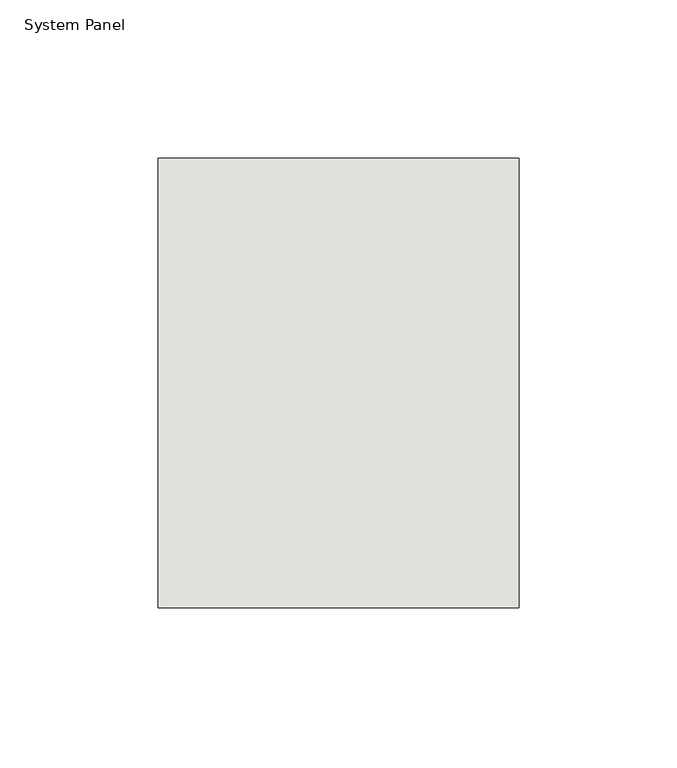
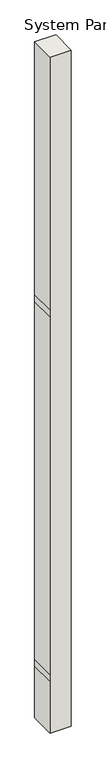
"""IFC4 building model written with IfcOpenShell, lengths in millimetres: wall geometry, System Panel : NLRS_21_CWP_hsb-vulling minerale wol 142 _gen_rsf."""

from ifc_helpers import new_model, si_unit, frame, origin, place, context, project, spatial, polyline, outline, extrude, source, transform, mapped, element, save


def system_panel_2185679e(model_context):
    return source(origin(), model_context, "Body", "SweptSolid", [
        extrude(outline(polyline([(0.0, -56.9999998), (0.0, 56.9999998), (295.0, 56.9999998), (333.0, 56.9999998), (2371.0, 56.9999998), (2409.0, 56.9999998), (3849.0, 56.9999998), (3849.0, -56.9999998), (2409.0, -56.9999998), (2371.0, -56.9999998), (333.0, -56.9999998), (295.0, -56.9999998), (0.0, -56.9999998)])), frame((0.0, -71.0, 0.0), z_axis=(0.0, 1.0, 0.0), x_axis=(0.0, 0.0, 1.0)), (0.0, 0.0, 1.0), 142.0),
    ])


if __name__ == "__main__":
    model = new_model("IFC4")
    model_context = context("Model", 3, world=origin())
    ifc_project = project(units=[si_unit("LENGTHUNIT", "METRE", prefix="MILLI")], contexts=[model_context])
    site = spatial("IfcSite", under=ifc_project)
    building = spatial("IfcBuilding", under=site)
    placement = place(None, origin())
    system_panel_shape = system_panel_2185679e(model_context)
    element("IfcWall", 1, ObjectType="System Panel : NLRS_21_CWP_hsb-vulling minerale wol 142 _gen_rsf", at=placement, inside=building, context=model_context, shape_type="MappedRepresentation", body=[
        mapped(system_panel_shape, transform((0.0, 0.0, 0.0), x_axis=(1.0, 0.0, 0.0), y_axis=(0.0, 1.0, 0.0), z_axis=(0.0, 0.0, 1.0))),
    ])
    save(model, "model.ifc")

# Revit data of these elements
# Type "System Panel : NLRS_21_CWP_hsb-vulling minerale wol 142 _gen_rsf"
#   Type IfcGUID = "07M7mRoiH1CR8m_RSKIwpC"
#   Assembly Code = "21.23"
#   IfcExportAs = "IfcWall"
# Element 1 (IfcWall, "System Panel : NLRS_21_CWP_hsb-vulling minerale wol 142 _gen_rsf")
#   Materials on its faces: "NLRS_m1_isolatie minerale wol_gen_rsf"
# Materials
#   "NLRS_m1_isolatie minerale wol_gen_rsf": class "M - Anorganische materialen", colour RGB 200 200 140, transparency 0, Keynote = "m1", Manufacturer = "Revit Standards Foundation", URL = "www.revitstandards.org", Description = "isolatie minerale wol", Cost = 0
